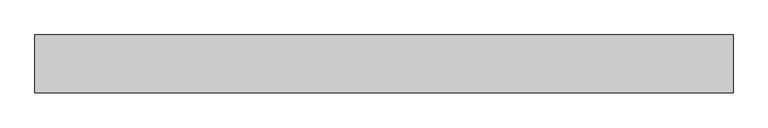
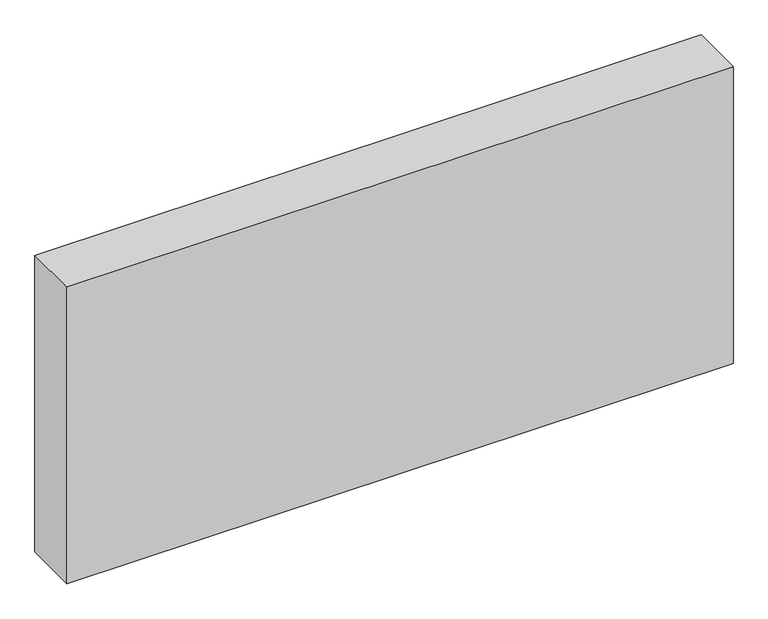
"""IFC4 building model written with IfcOpenShell, lengths in millimetres: proxy geometry, Generic Models 7:Generic Models 1:5:Generic Models 1:5 : Generic Models 7:Generic Models 1:337419:13 : Generic Models 7:Generic Models 1:5:Generic Models 1:5 : Generic Models 7:Generic Models 1:337419:311462."""

import ifcopenshell
import ifcopenshell.guid

model = None  # the IFC model being written
_history = None  # IfcOwnerHistory: only IFC2X3 demands one
_inside = {}  # id of a spatial element -> (the spatial element, [elements in it])
_under = {}  # id of a project, library or spatial element -> (it, [spatial elements below it])
_declared = {}  # id of a project -> (the project, [libraries it declares])
_typed = {}  # id of a type object -> (the type object, [elements of that type])
_made_of = {}  # id of a material, layer set ... -> (it, [elements and type objects made of it])


def new_model(schema):
    """Start an empty IFC model of exactly this schema.

    Asked for "IFC4X3", IfcOpenShell would pick the latest addendum, in which some entities
    have other attributes; the version numbers below select the first issue.
    IFC2X3 requires an IfcOwnerHistory on every rooted entity: one is made here for all.
    """
    global model, _history
    if schema == "IFC4X3":
        model = ifcopenshell.file(schema_version=(4, 3, 0, 0))
    else:
        model = ifcopenshell.file(schema=schema)
    _inside.clear()
    _under.clear()
    _declared.clear()
    _typed.clear()
    _made_of.clear()
    _history = None
    if model.schema == "IFC2X3":
        org = make("IfcOrganization", Name="unknown")
        user = make(
            "IfcPersonAndOrganization",
            ThePerson=make("IfcPerson", FamilyName="unknown"),
            TheOrganization=org,
        )
        app = make(
            "IfcApplication",
            ApplicationDeveloper=org,
            Version="unknown",
            ApplicationFullName="unknown",
            ApplicationIdentifier="unknown",
        )
        _history = make(
            "IfcOwnerHistory",
            OwningUser=user,
            OwningApplication=app,
            ChangeAction="ADDED",
            CreationDate=0,
        )
    return model


def make(cls, **values):
    """One entity of the class cls with the attributes given. An attribute that is None is left unset."""
    return model.create_entity(
        cls, **{name: value for name, value in values.items() if value is not None}
    )


def rooted(cls, **values):
    """An entity with a GlobalId (a new one), such as an element, a storey or a relation."""
    return make(cls, GlobalId=ifcopenshell.guid.new(), OwnerHistory=_history, **values)


def si_unit(unit_type, name, prefix=None):
    """IfcSIUnit, for example si_unit("LENGTHUNIT", "METRE", prefix="MILLI")."""
    return make("IfcSIUnit", UnitType=unit_type, Prefix=prefix, Name=name)


def assignment(units):
    """IfcUnitAssignment: the units of a project."""
    return None if units is None else make("IfcUnitAssignment", Units=units)


def point(xyz):
    """IfcCartesianPoint."""
    return None if xyz is None else make("IfcCartesianPoint", Coordinates=xyz)


def direction(xyz):
    """IfcDirection."""
    return None if xyz is None else make("IfcDirection", DirectionRatios=xyz)


def frame(location, z_axis=None, x_axis=None):
    """IfcAxis2Placement3D, a coordinate frame: its origin and axes. An axis left out is left unset."""
    return make(
        "IfcAxis2Placement3D",
        Location=point(location),
        Axis=direction(z_axis),
        RefDirection=direction(x_axis),
    )


def origin():
    """The frame at (0, 0, 0) with its axes left unset."""
    return frame((0.0, 0.0, 0.0))


def place(relative_to, where):
    """IfcLocalPlacement: puts the frame where relative to a parent placement (None: the world)."""
    return make(
        "IfcLocalPlacement", PlacementRelTo=relative_to, RelativePlacement=where
    )


def context(
    kind, dimensions, precision=None, world=None, true_north=None, identifier=None
):
    """IfcGeometricRepresentationContext, for example the 3D "Model" context."""
    return make(
        "IfcGeometricRepresentationContext",
        ContextIdentifier=identifier,
        ContextType=kind,
        CoordinateSpaceDimension=dimensions,
        Precision=precision,
        WorldCoordinateSystem=world,
        TrueNorth=true_north,
    )


def project(units=None, contexts=None):
    """IfcProject with its units and contexts."""
    return rooted(
        "IfcProject",
        Name="project",
        RepresentationContexts=contexts,
        UnitsInContext=assignment(units),
    )


def spatial(cls, under=None, at=None, **own):
    """A site, building, storey or space (cls), placed at a placement, below another one or the project."""
    s = rooted(cls, ObjectPlacement=at, **own)
    if under is not None:
        _under.setdefault(under.id(), (under, []))[1].append(s)
    return s


def polyline(points):
    """IfcPolyline through the points."""
    return make("IfcPolyline", Points=[point(p) for p in points])


def outline(outer, holes=None, kind="AREA"):
    """IfcArbitraryClosedProfileDef: a profile drawn as a closed curve; with holes, ...WithVoids."""
    if holes is None:
        return make("IfcArbitraryClosedProfileDef", ProfileType=kind, OuterCurve=outer)
    return make(
        "IfcArbitraryProfileDefWithVoids",
        ProfileType=kind,
        OuterCurve=outer,
        InnerCurves=holes,
    )


def extrude(swept, where, along, depth):
    """IfcExtrudedAreaSolid: the profile swept, set in the frame where, extruded along a direction by depth."""
    return make(
        "IfcExtrudedAreaSolid",
        SweptArea=swept,
        Position=where,
        ExtrudedDirection=direction(along),
        Depth=depth,
    )


def shape(context_of_items, identifier, shape_type, items):
    """IfcShapeRepresentation: the items that make up one representation, for example the "Body"."""
    return make(
        "IfcShapeRepresentation",
        ContextOfItems=context_of_items,
        RepresentationIdentifier=identifier,
        RepresentationType=shape_type,
        Items=items,
    )


def source(mapping_origin, context_of_items, identifier, shape_type, items):
    """IfcRepresentationMap: a shape defined once, which mapped items show again and again."""
    return make(
        "IfcRepresentationMap",
        MappingOrigin=mapping_origin,
        MappedRepresentation=shape(context_of_items, identifier, shape_type, items),
    )


def transform(
    local_origin,
    x_axis=None,
    y_axis=None,
    z_axis=None,
    scale=None,
    scale2=None,
    scale3=None,
    uniform=True,
):
    """IfcCartesianTransformationOperator3D, or its non-uniform kind. x_axis, y_axis, z_axis: its Axis1, 2, 3."""
    if uniform:
        return make(
            "IfcCartesianTransformationOperator3D",
            Axis1=direction(x_axis),
            Axis2=direction(y_axis),
            LocalOrigin=point(local_origin),
            Scale=scale,
            Axis3=direction(z_axis),
        )
    return make(
        "IfcCartesianTransformationOperator3DnonUniform",
        Axis1=direction(x_axis),
        Axis2=direction(y_axis),
        LocalOrigin=point(local_origin),
        Scale=scale,
        Axis3=direction(z_axis),
        Scale2=scale2,
        Scale3=scale3,
    )


def mapped(mapping_source, mapping_target):
    """IfcMappedItem: shows the shape of a source again, moved by a transform."""
    return make(
        "IfcMappedItem", MappingSource=mapping_source, MappingTarget=mapping_target
    )


def made_of(thing, what):
    """Note that an element or type object is made of a material, layer set ...; save() writes the relation."""
    if what is not None:
        _made_of.setdefault(what.id(), (what, []))[1].append(thing)
    return thing


def element(
    cls,
    number,
    at=None,
    inside=None,
    cuts=None,
    type_object=None,
    material=None,
    context=None,
    identifier="Body",
    shape_type=None,
    held_by="IfcProductDefinitionShape",
    body=None,
    shapes=None,
    **own,
):
    """One element of the class cls, such as IfcWall. Its Tag is "e" and its number.

    at: its placement. inside: the storey or other place that contains it. cuts: it is an
    opening in that element (IfcRelVoidsElement). A single representation is given by context,
    identifier, shape_type and body (its items); several are given by shapes. held_by: the class
    of the entity that holds the representations. save() writes the other relations.
    """
    e = rooted(cls, Tag="e%d" % number, ObjectPlacement=at, **own)
    if body is not None:
        shapes = [shape(context, identifier, shape_type, body)]
    if shapes is not None:
        e.Representation = make(held_by, Representations=shapes)
    if inside is not None:
        _inside.setdefault(inside.id(), (inside, []))[1].append(e)
    if cuts is not None:
        rooted(
            "IfcRelVoidsElement", RelatingBuildingElement=cuts, RelatedOpeningElement=e
        )
    if type_object is not None:
        _typed.setdefault(type_object.id(), (type_object, []))[1].append(e)
    return made_of(e, material)


def aggregate(whole, parts):
    """IfcRelAggregates: a whole, such as a stair, and the parts it consists of."""
    return rooted("IfcRelAggregates", RelatingObject=whole, RelatedObjects=parts)


def save(model, path):
    """Write the relations noted so far, then the file.

    IfcRelAggregates (storeys below a building ...), IfcRelContainedInSpatialStructure (elements
    in a storey), IfcRelDefinesByType, IfcRelAssociatesMaterial and IfcRelDeclares: one each for
    every whole, place, type object, material and project.
    """
    for whole, parts in _under.values():
        aggregate(whole, parts)
    for where, things in _inside.values():
        rooted(
            "IfcRelContainedInSpatialStructure",
            RelatedElements=things,
            RelatingStructure=where,
        )
    for kind, things in _typed.values():
        rooted("IfcRelDefinesByType", RelatedObjects=things, RelatingType=kind)
    for what, things in _made_of.values():
        rooted("IfcRelAssociatesMaterial", RelatedObjects=things, RelatingMaterial=what)
    for by, libraries in _declared.values():
        rooted("IfcRelDeclares", RelatingContext=by, RelatedDefinitions=libraries)
    model.write(path)


def generic_models_fdadf2c7(model_context):
    return source(origin(), model_context, "Body", "SweptSolid", [
        extrude(outline(polyline([(572897.3867239, -578799.0788841), (572897.3867239, -578999.1038841), (570490.7367239, -578999.1038841), (570490.7367239, -578799.0788841), (572897.3867239, -578799.0788841)])), frame((0.0, 0.0, 1311.0765625), z_axis=(0.0, 0.0, 1.0), x_axis=(1.0, 0.0, 0.0)), (0.0, 0.0, 1.0), 1133.871875),
    ])


if __name__ == "__main__":
    model = new_model("IFC4")
    model_context = context("Model", 3, world=origin())
    ifc_project = project(units=[si_unit("LENGTHUNIT", "METRE", prefix="MILLI")], contexts=[model_context])
    site = spatial("IfcSite", under=ifc_project)
    building = spatial("IfcBuilding", under=site)
    placement = place(None, origin())
    generic_models_shape = generic_models_fdadf2c7(model_context)
    element("IfcBuildingElementProxy", 1, Name="Generic Models 7:Generic Models 1:5:Generic Models 1:5 : Generic Models 7:Generic Models 1:337419:13 : Generic Models 7:Generic Models 1:5:Generic Models 1:5 : Generic Models 7:Generic Models 1:337419:311462", ObjectType="Generic Models 7:Generic Models 1:5:Generic Models 1:5 : Generic Models 7:Generic Models 1:337419:13 : Generic Models 7:Generic Models 1:5:Generic Models 1:5 : Generic Models 7:Generic Models 1:337419:311462", at=placement, inside=building, context=model_context, shape_type="MappedRepresentation", body=[
        mapped(generic_models_shape, transform((0.0, 0.0, 0.0), x_axis=(1.0, 0.0, 0.0), y_axis=(0.0, 1.0, 0.0), z_axis=(0.0, 0.0, 1.0))),
    ])
    save(model, "model.ifc")

# Revit data of these elements
# Type "Generic Models 7:Generic Models 1:5:Generic Models 1:5 : Generic Models 7:Generic Models 1:337419:13 : Generic Models 7:Generic Models 1:5:Generic Models 1:5 : Generic Models 7:Generic Models 1:337419:311462"
#   NameOverride = "Generic Models 7:Generic Models 1:5:Generic Models 1:5 : Generic Models 7:Generic Models 1:337419:311462"
#   ObjectTypeOverride = "Generic Models 1:5 : Generic Models 7:Generic Models 1:337419"
#   Reference = "Generic Models 1"
#   Tag = "311462"
